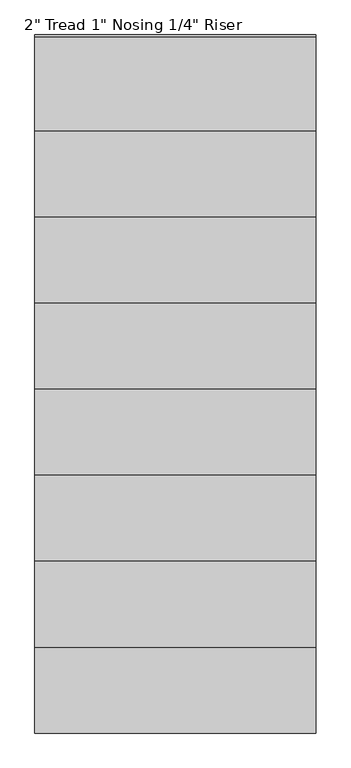
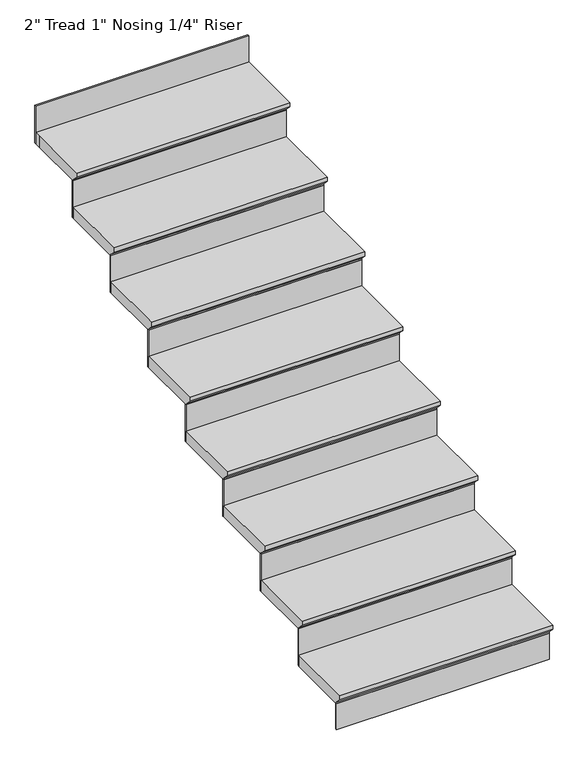
"""IFC4 building model written with IfcOpenShell, lengths in millimetres: stair flight geometry."""

from ifc_helpers import new_model, si_unit, origin, place, context, project, spatial, faceted_brep, source, transform, mapped, element, save


def stair_flight_a8b112ed(model_context):
    return source(origin(), model_context, "Body", "Brep", [
        faceted_brep([(15827.5123343, 14886.0483822, 150.2833333), (15827.5123343, 14886.0483822, 169.3333333), (14913.1123343, 14886.0483822, 169.3333333), (14913.1123343, 14886.0483822, 150.2833333), (15827.5123343, 14911.4483822, 124.8833333), (14913.1123343, 14911.4483822, 124.8833333), (15827.5123343, 15190.8483822, 169.3333333), (14913.1123343, 15190.8483822, 169.3333333), (14913.1123343, 14911.4483822, 118.5333333), (14913.1123343, 15190.8483822, 118.5333333), (15827.5123343, 15190.8483822, 118.5333333), (15827.5123343, 14911.4483822, 118.5333333)], [[[0, 1, 2, 3]], [[4, 0, 3, 5]], [[2, 1, 6, 7]], [[8, 9, 10, 11]], [[2, 7, 9, 8, 5, 3]], [[8, 11, 4, 5]], [[6, 1, 0, 4, 11, 10]], [[7, 6, 10, 9]]]),
        faceted_brep([(15827.5123343, 14911.4483822, 118.5333333), (15827.5123343, 14911.4483822, 0.0), (15827.5123343, 14917.7983822, 0.0), (15827.5123343, 14917.7983822, 118.5333333), (14913.1123343, 14911.4483822, 118.5333333), (14913.1123343, 14917.7983822, 118.5333333), (14913.1123343, 14917.7983822, 0.0), (14913.1123343, 14911.4483822, 0.0)], [[[0, 1, 2, 3]], [[4, 5, 6, 7]], [[1, 0, 4, 7]], [[2, 1, 7, 6]], [[3, 2, 6, 5]], [[0, 3, 5, 4]]]),
        faceted_brep([(15827.5123343, 15190.8483822, 287.8666667), (15827.5123343, 15190.8483822, 118.5333333), (15827.5123343, 15197.1983822, 118.5333333), (15827.5123343, 15197.1983822, 287.8666667), (14913.1123343, 15190.8483822, 287.8666667), (14913.1123343, 15197.1983822, 287.8666667), (14913.1123343, 15197.1983822, 118.5333333), (14913.1123343, 15190.8483822, 118.5333333)], [[[0, 1, 2, 3]], [[4, 5, 6, 7]], [[1, 0, 4, 7]], [[2, 1, 7, 6]], [[3, 2, 6, 5]], [[0, 3, 5, 4]]]),
        faceted_brep([(14913.1123343, 15165.4483822, 338.6666667), (15827.5123343, 15165.4483822, 338.6666667), (15827.5123343, 15470.2483822, 338.6666667), (14913.1123343, 15470.2483822, 338.6666667), (14913.1123343, 15190.8483822, 287.8666667), (14913.1123343, 15470.2483822, 287.8666667), (15827.5123343, 15470.2483822, 287.8666667), (15827.5123343, 15190.8483822, 287.8666667), (14913.1123343, 15190.8483822, 294.2166667), (14913.1123343, 15165.4483822, 319.6166667), (15827.5123343, 15190.8483822, 294.2166667), (15827.5123343, 15165.4483822, 319.6166667)], [[[0, 1, 2, 3]], [[4, 5, 6, 7]], [[0, 3, 5, 4, 8, 9]], [[4, 7, 10, 8]], [[2, 1, 11, 10, 7, 6]], [[3, 2, 6, 5]], [[11, 1, 0, 9]], [[10, 11, 9, 8]]]),
        faceted_brep([(15827.5123343, 15470.2483822, 457.2), (15827.5123343, 15470.2483822, 287.8666667), (15827.5123343, 15476.5983822, 287.8666667), (15827.5123343, 15476.5983822, 457.2), (14913.1123343, 15470.2483822, 457.2), (14913.1123343, 15476.5983822, 457.2), (14913.1123343, 15476.5983822, 287.8666667), (14913.1123343, 15470.2483822, 287.8666667)], [[[0, 1, 2, 3]], [[4, 5, 6, 7]], [[1, 0, 4, 7]], [[2, 1, 7, 6]], [[3, 2, 6, 5]], [[0, 3, 5, 4]]]),
        faceted_brep([(14913.1123343, 15444.8483822, 508.0), (15827.5123343, 15444.8483822, 508.0), (15827.5123343, 15749.6483822, 508.0), (14913.1123343, 15749.6483822, 508.0), (14913.1123343, 15470.2483822, 457.2), (14913.1123343, 15749.6483822, 457.2), (15827.5123343, 15749.6483822, 457.2), (15827.5123343, 15470.2483822, 457.2), (14913.1123343, 15470.2483822, 463.55), (14913.1123343, 15444.8483822, 488.95), (15827.5123343, 15470.2483822, 463.55), (15827.5123343, 15444.8483822, 488.95)], [[[0, 1, 2, 3]], [[4, 5, 6, 7]], [[0, 3, 5, 4, 8, 9]], [[4, 7, 10, 8]], [[2, 1, 11, 10, 7, 6]], [[3, 2, 6, 5]], [[11, 1, 0, 9]], [[10, 11, 9, 8]]]),
        faceted_brep([(15827.5123343, 15749.6483822, 626.5333333), (15827.5123343, 15749.6483822, 457.2), (15827.5123343, 15755.9983822, 457.2), (15827.5123343, 15755.9983822, 626.5333333), (14913.1123343, 15749.6483822, 626.5333333), (14913.1123343, 15755.9983822, 626.5333333), (14913.1123343, 15755.9983822, 457.2), (14913.1123343, 15749.6483822, 457.2)], [[[0, 1, 2, 3]], [[4, 5, 6, 7]], [[1, 0, 4, 7]], [[2, 1, 7, 6]], [[3, 2, 6, 5]], [[0, 3, 5, 4]]]),
        faceted_brep([(14913.1123343, 15724.2483822, 677.3333333), (15827.5123343, 15724.2483822, 677.3333333), (15827.5123343, 16029.0483822, 677.3333333), (14913.1123343, 16029.0483822, 677.3333333), (14913.1123343, 15749.6483822, 626.5333333), (14913.1123343, 16029.0483822, 626.5333333), (15827.5123343, 16029.0483822, 626.5333333), (15827.5123343, 15749.6483822, 626.5333333), (14913.1123343, 15749.6483822, 632.8833333), (14913.1123343, 15724.2483822, 658.2833333), (15827.5123343, 15749.6483822, 632.8833333), (15827.5123343, 15724.2483822, 658.2833333)], [[[0, 1, 2, 3]], [[4, 5, 6, 7]], [[0, 3, 5, 4, 8, 9]], [[4, 7, 10, 8]], [[2, 1, 11, 10, 7, 6]], [[3, 2, 6, 5]], [[11, 1, 0, 9]], [[10, 11, 9, 8]]]),
        faceted_brep([(15827.5123343, 16029.0483822, 795.8666667), (15827.5123343, 16029.0483822, 626.5333333), (15827.5123343, 16035.3983822, 626.5333333), (15827.5123343, 16035.3983822, 795.8666667), (14913.1123343, 16029.0483822, 795.8666667), (14913.1123343, 16035.3983822, 795.8666667), (14913.1123343, 16035.3983822, 626.5333333), (14913.1123343, 16029.0483822, 626.5333333)], [[[0, 1, 2, 3]], [[4, 5, 6, 7]], [[1, 0, 4, 7]], [[2, 1, 7, 6]], [[3, 2, 6, 5]], [[0, 3, 5, 4]]]),
        faceted_brep([(14913.1123343, 16003.6483822, 846.6666667), (15827.5123343, 16003.6483822, 846.6666667), (15827.5123343, 16308.4483822, 846.6666667), (14913.1123343, 16308.4483822, 846.6666667), (14913.1123343, 16029.0483822, 795.8666667), (14913.1123343, 16308.4483822, 795.8666667), (15827.5123343, 16308.4483822, 795.8666667), (15827.5123343, 16029.0483822, 795.8666667), (14913.1123343, 16029.0483822, 802.2166667), (14913.1123343, 16003.6483822, 827.6166667), (15827.5123343, 16029.0483822, 802.2166667), (15827.5123343, 16003.6483822, 827.6166667)], [[[0, 1, 2, 3]], [[4, 5, 6, 7]], [[0, 3, 5, 4, 8, 9]], [[4, 7, 10, 8]], [[2, 1, 11, 10, 7, 6]], [[3, 2, 6, 5]], [[11, 1, 0, 9]], [[10, 11, 9, 8]]]),
        faceted_brep([(15827.5123343, 16308.4483822, 965.2), (15827.5123343, 16308.4483822, 795.8666667), (15827.5123343, 16314.7983822, 795.8666667), (15827.5123343, 16314.7983822, 965.2), (14913.1123343, 16308.4483822, 965.2), (14913.1123343, 16314.7983822, 965.2), (14913.1123343, 16314.7983822, 795.8666667), (14913.1123343, 16308.4483822, 795.8666667)], [[[0, 1, 2, 3]], [[4, 5, 6, 7]], [[1, 0, 4, 7]], [[2, 1, 7, 6]], [[3, 2, 6, 5]], [[0, 3, 5, 4]]]),
        faceted_brep([(14913.1123343, 16283.0483822, 1016.0), (15827.5123343, 16283.0483822, 1016.0), (15827.5123343, 16587.8483822, 1016.0), (14913.1123343, 16587.8483822, 1016.0), (14913.1123343, 16308.4483822, 965.2), (14913.1123343, 16587.8483822, 965.2), (15827.5123343, 16587.8483822, 965.2), (15827.5123343, 16308.4483822, 965.2), (14913.1123343, 16308.4483822, 971.55), (14913.1123343, 16283.0483822, 996.95), (15827.5123343, 16308.4483822, 971.55), (15827.5123343, 16283.0483822, 996.95)], [[[0, 1, 2, 3]], [[4, 5, 6, 7]], [[0, 3, 5, 4, 8, 9]], [[4, 7, 10, 8]], [[2, 1, 11, 10, 7, 6]], [[3, 2, 6, 5]], [[11, 1, 0, 9]], [[10, 11, 9, 8]]]),
        faceted_brep([(15827.5123343, 16587.8483822, 1134.5333333), (15827.5123343, 16587.8483822, 965.2), (15827.5123343, 16594.1983822, 965.2), (15827.5123343, 16594.1983822, 1134.5333333), (14913.1123343, 16587.8483822, 1134.5333333), (14913.1123343, 16594.1983822, 1134.5333333), (14913.1123343, 16594.1983822, 965.2), (14913.1123343, 16587.8483822, 965.2)], [[[0, 1, 2, 3]], [[4, 5, 6, 7]], [[1, 0, 4, 7]], [[2, 1, 7, 6]], [[3, 2, 6, 5]], [[0, 3, 5, 4]]]),
        faceted_brep([(14913.1123343, 16562.4483822, 1185.3333333), (15827.5123343, 16562.4483822, 1185.3333333), (15827.5123343, 16867.2483822, 1185.3333333), (14913.1123343, 16867.2483822, 1185.3333333), (14913.1123343, 16587.8483822, 1134.5333333), (14913.1123343, 16867.2483822, 1134.5333333), (15827.5123343, 16867.2483822, 1134.5333333), (15827.5123343, 16587.8483822, 1134.5333333), (14913.1123343, 16587.8483822, 1140.8833333), (14913.1123343, 16562.4483822, 1166.2833333), (15827.5123343, 16587.8483822, 1140.8833333), (15827.5123343, 16562.4483822, 1166.2833333)], [[[0, 1, 2, 3]], [[4, 5, 6, 7]], [[0, 3, 5, 4, 8, 9]], [[4, 7, 10, 8]], [[2, 1, 11, 10, 7, 6]], [[3, 2, 6, 5]], [[11, 1, 0, 9]], [[10, 11, 9, 8]]]),
        faceted_brep([(15827.5123343, 17146.6483822, 1473.2), (15827.5123343, 17146.6483822, 1303.8666667), (15827.5123343, 17152.9983822, 1303.8666667), (15827.5123343, 17152.9983822, 1473.2), (14913.1123343, 17146.6483822, 1473.2), (14913.1123343, 17152.9983822, 1473.2), (14913.1123343, 17152.9983822, 1303.8666667), (14913.1123343, 17146.6483822, 1303.8666667)], [[[0, 1, 2, 3]], [[4, 5, 6, 7]], [[1, 0, 4, 7]], [[2, 1, 7, 6]], [[3, 2, 6, 5]], [[0, 3, 5, 4]]]),
        faceted_brep([(15827.5123343, 16867.2483822, 1303.8666667), (15827.5123343, 16867.2483822, 1134.5333333), (15827.5123343, 16873.5983822, 1134.5333333), (15827.5123343, 16873.5983822, 1303.8666667), (14913.1123343, 16867.2483822, 1303.8666667), (14913.1123343, 16873.5983822, 1303.8666667), (14913.1123343, 16873.5983822, 1134.5333333), (14913.1123343, 16867.2483822, 1134.5333333)], [[[0, 1, 2, 3]], [[4, 5, 6, 7]], [[1, 0, 4, 7]], [[2, 1, 7, 6]], [[3, 2, 6, 5]], [[0, 3, 5, 4]]]),
        faceted_brep([(14913.1123343, 17146.6483822, 1354.6666667), (14913.1123343, 17121.2483822, 1354.6666667), (14913.1123343, 16841.8483822, 1354.6666667), (15827.5123343, 16841.8483822, 1354.6666667), (15827.5123343, 17146.6483822, 1354.6666667), (14913.1123343, 17121.2483822, 1303.8666667), (14913.1123343, 17146.6483822, 1303.8666667), (15827.5123343, 17146.6483822, 1303.8666667), (15827.5123343, 16867.2483822, 1303.8666667), (14913.1123343, 16867.2483822, 1303.8666667), (14913.1123343, 16867.2483822, 1310.2166667), (14913.1123343, 16841.8483822, 1335.6166667), (15827.5123343, 16867.2483822, 1310.2166667), (15827.5123343, 16841.8483822, 1335.6166667)], [[[0, 1, 2, 3, 4]], [[5, 6, 7, 8, 9]], [[1, 0, 6, 5]], [[2, 1, 5, 9, 10, 11]], [[9, 8, 12, 10]], [[4, 3, 13, 12, 8, 7]], [[0, 4, 7, 6]], [[13, 3, 2, 11]], [[12, 13, 11, 10]]]),
    ])


if __name__ == "__main__":
    model = new_model("IFC4")
    model_context = context("Model", 3, world=origin())
    ifc_project = project(units=[si_unit("LENGTHUNIT", "METRE", prefix="MILLI")], contexts=[model_context])
    site = spatial("IfcSite", under=ifc_project)
    building = spatial("IfcBuilding", under=site)
    placement = place(None, origin())
    stair_flight_shape = stair_flight_a8b112ed(model_context)
    element("IfcStairFlight", 1, ObjectType="2\" Tread 1\" Nosing 1/4\" Riser", at=placement, inside=building, context=model_context, shape_type="MappedRepresentation", body=[
        mapped(stair_flight_shape, transform((0.0, 0.0, 0.0), x_axis=(1.0, 0.0, 0.0), y_axis=(0.0, 1.0, 0.0), z_axis=(0.0, 0.0, 1.0))),
    ])
    save(model, "model.ifc")
